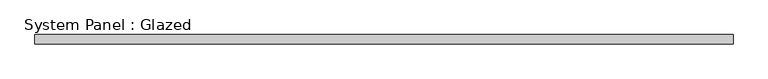
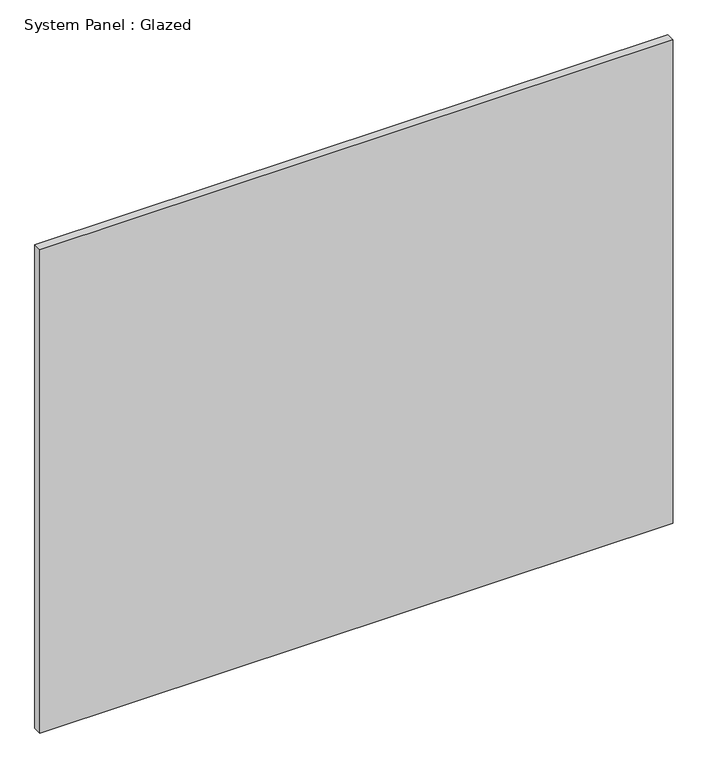
"""IFC4 building model written with IfcOpenShell, lengths in millimetres: plate geometry, System Panel : Glazed."""

from ifc_helpers import new_model, si_unit, origin, origin_with_axes, place, context, project, spatial, polyline, outline, extrude, source, transform, mapped, element, save


def system_panel_glazed_382e80de(model_context):
    return source(origin(), model_context, "Body", "SweptSolid", [
        extrude(outline(polyline([(915.0000002, 24.5), (-915.0000002, 24.5), (-915.0000002, 49.5), (915.0000002, 49.5), (915.0000002, 24.5)])), origin_with_axes(), (0.0, 0.0, 1.0), 1476.6044889),
    ])


if __name__ == "__main__":
    model = new_model("IFC4")
    model_context = context("Model", 3, world=origin())
    ifc_project = project(units=[si_unit("LENGTHUNIT", "METRE", prefix="MILLI")], contexts=[model_context])
    site = spatial("IfcSite", under=ifc_project)
    building = spatial("IfcBuilding", under=site)
    placement = place(None, origin())
    system_panel_glazed_shape = system_panel_glazed_382e80de(model_context)
    element("IfcPlate", 1, ObjectType="System Panel : Glazed", at=placement, inside=building, context=model_context, shape_type="MappedRepresentation", body=[
        mapped(system_panel_glazed_shape, transform((0.0, 0.0, 0.0), x_axis=(1.0, 0.0, 0.0), y_axis=(0.0, 1.0, 0.0), z_axis=(0.0, 0.0, 1.0))),
    ])
    save(model, "model.ifc")

# Revit data of these elements
# Element 1 (IfcPlate, "System Panel : Glazed")
#   Materials on its faces: "Glass"
# Materials
#   "Glass": class "Glass", colour RGB 218 227 224, transparency 0.85, Description = "Soda Lime Glass", Cost = 0
